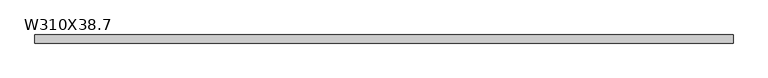
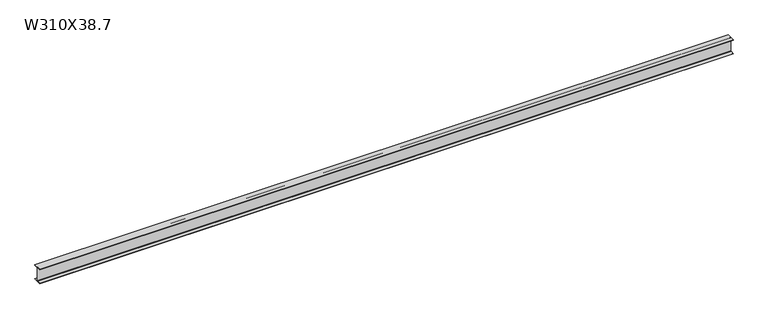
"""IFC4 building model written with IfcOpenShell, lengths in millimetres: beam geometry, M_W Shapes : W310X38.7."""

from ifc_helpers import new_model, si_unit, point, frame, frame_2d, origin, place, context, project, spatial, polyline, circle_curve, trimmed, segment, composite_curve, outline, extrude, source, transform, mapped, element, save


def w310x38_7_8ffbaecc(model_context):
    return source(origin(), model_context, "Body", "SweptSolid", [
        extrude(outline(composite_curve([segment(polyline([(82.5, -145.35), (82.5, -155.0), (-82.5, -155.0), (-82.5, -145.35), (-10.57, -145.35)]), True, "CONTINUOUS"), segment(trimmed(circle_curve(frame_2d((-10.57, -137.7)), 7.65), [point((-10.57, -145.35))], [point((-2.92, -137.7))], True, "CARTESIAN"), True, "CONTINUOUS"), segment(polyline([(-2.92, -137.7), (-2.92, 137.7)]), True, "CONTINUOUS"), segment(trimmed(circle_curve(frame_2d((-10.57, 137.7)), 7.65), [point((-2.92, 137.7))], [point((-10.57, 145.35))], True, "CARTESIAN"), True, "CONTINUOUS"), segment(polyline([(-10.57, 145.35), (-82.5, 145.35), (-82.5, 155.0), (82.5, 155.0), (82.5, 145.35), (10.57, 145.35)]), True, "CONTINUOUS"), segment(trimmed(circle_curve(frame_2d((10.57, 137.7)), 7.65), [point((10.57, 145.35))], [point((2.92, 137.7))], True, "CARTESIAN"), True, "CONTINUOUS"), segment(polyline([(2.92, 137.7), (2.92, -137.7)]), True, "CONTINUOUS"), segment(trimmed(circle_curve(frame_2d((10.57, -137.7)), 7.65), [point((2.92, -137.7))], [point((10.57, -145.35))], True, "CARTESIAN"), True, "CONTINUOUS"), segment(polyline([(10.57, -145.35), (82.5, -145.35)]), True, "CONTINUOUS")], self_intersect=False)), frame((-7096.65, 0.0, 0.0), z_axis=(1.0, 0.0, 0.0), x_axis=(0.0, 1.0, 0.0)), (0.0, 0.0, 1.0), 14119.9),
    ])


if __name__ == "__main__":
    model = new_model("IFC4")
    model_context = context("Model", 3, world=origin())
    ifc_project = project(units=[si_unit("LENGTHUNIT", "METRE", prefix="MILLI")], contexts=[model_context])
    site = spatial("IfcSite", under=ifc_project)
    building = spatial("IfcBuilding", under=site)
    placement = place(None, origin())
    w310x38_7_shape = w310x38_7_8ffbaecc(model_context)
    element("IfcBeam", 1, ObjectType="M_W Shapes : W310X38.7", at=placement, inside=building, context=model_context, shape_type="MappedRepresentation", body=[
        mapped(w310x38_7_shape, transform((0.0, 0.0, 0.0), x_axis=(1.0, 0.0, 0.0), y_axis=(0.0, 1.0, 0.0), z_axis=(0.0, 0.0, 1.0))),
    ])
    save(model, "model.ifc")

# Revit data of these elements
# Type "M_W Shapes : W310X38.7"
#   Section Name Key = "W12x26"
#   Width = 165 mm
#   Web Thickness = 5.84 mm
#   Web Fillet = 7.65 mm
#   Warping Constant = 163000 cm⁶
#   Torsional Moment of Inertia = 12.5 cm⁴
#   Section Area = 49.4 cm²
#   Plastic Modulus weak axis = 0.00473217 (stored number, unit not read)
#   Plastic Modulus strong axis = 0.0215419 (stored number, unit not read)
#   Perimeter = 1.25 m²/m
#   Nominal Weight = 379.516 N/m
#   Moment of Inertia weak axis = 720 cm⁴
#   Moment of Inertia strong axis = 8490 cm⁴
#   Height = 310 mm
#   Flange Thickness = 9.65 mm
#   Elastic Modulus weak axis = 0.00309003 (stored number, unit not read)
#   Elastic Modulus strong axis = 0.0193171 (stored number, unit not read)
#   Centroid Vertical = 155 mm
#   Centroid Horizontal = 82.5 mm
#   Length [instance default] = 1.5 m
#   Structural Material [instance default] = Steel, 45-345
#   Assembly Code = ""
# Element 1 (IfcBeam, "M_W Shapes : W310X38.7")
#   Materials on its faces: "Steel, 45-345"
# Materials
#   "Steel, 45-345": class "Metal", colour RGB 189 187 185, transparency 0, Description = "Steel 345 MPa", Cost = 0
